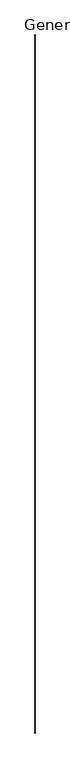
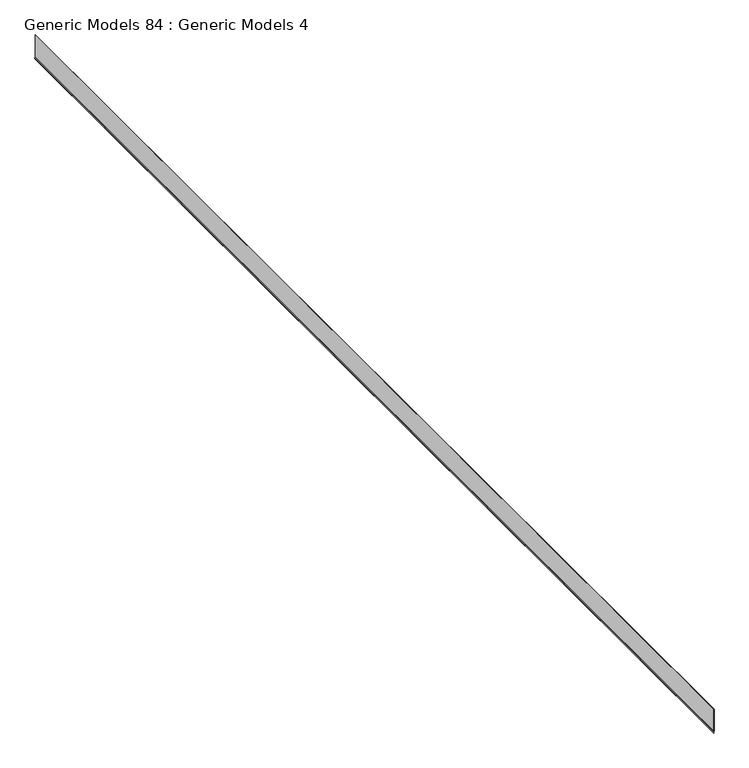
"""IFC4 building model written with IfcOpenShell, lengths in millimetres: proxy geometry, Generic Models 84 : Generic Models 4."""

from ifc_helpers import new_model, si_unit, frame, origin, place, context, project, spatial, polyline, outline, extrude, source, transform, mapped, element, save


def generic_models_84_generic_models_4_ea4e6b37(model_context):
    return source(origin(), model_context, "Body", "SweptSolid", [
        extrude(outline(polyline([(126371.6156249, -8345.4097752), (126742.9877991, -8345.4097752), (126742.9877991, -8346.2035252), (126371.7555845, -8346.2035252), (126360.6618382, -8350.2413186), (126345.6080757, -8350.2413186), (126345.6080757, -8349.4475686), (126360.5218787, -8349.4475686), (126371.6156249, -8345.4097752)])), frame((0.0, -6864.9230338, 0.0), z_axis=(0.0, 1.0, 0.0), x_axis=(0.0, 0.0, 1.0)), (0.0, 0.0, 1.0), 18643.6),
    ])


if __name__ == "__main__":
    model = new_model("IFC4")
    model_context = context("Model", 3, world=origin())
    ifc_project = project(units=[si_unit("LENGTHUNIT", "METRE", prefix="MILLI")], contexts=[model_context])
    site = spatial("IfcSite", under=ifc_project)
    building = spatial("IfcBuilding", under=site)
    placement = place(None, origin())
    generic_models_84_generic_models_4_shape = generic_models_84_generic_models_4_ea4e6b37(model_context)
    element("IfcBuildingElementProxy", 1, Name="Generic Models 84 : Generic Models 4", ObjectType="Generic Models 84 : Generic Models 4", at=placement, inside=building, context=model_context, shape_type="MappedRepresentation", body=[
        mapped(generic_models_84_generic_models_4_shape, transform((0.0, 0.0, 0.0), x_axis=(1.0, 0.0, 0.0), y_axis=(0.0, 1.0, 0.0), z_axis=(0.0, 0.0, 1.0))),
    ])
    save(model, "model.ifc")

# Revit data of these elements
# Element 1 (IfcBuildingElementProxy, "Generic Models 84 : Generic Models 4")
#   Materials on its faces: "_(2) LAYERS NO. 30 ASTM D226 ASPHALT SATURATED ORGANIC FELT"
# Materials
#   "_(2) LAYERS NO. 30 ASTM D226 ASPHALT SATURATED ORGANIC FELT": class "Generic", colour RGB 67 154 161, transparency 0, Cost = 0
